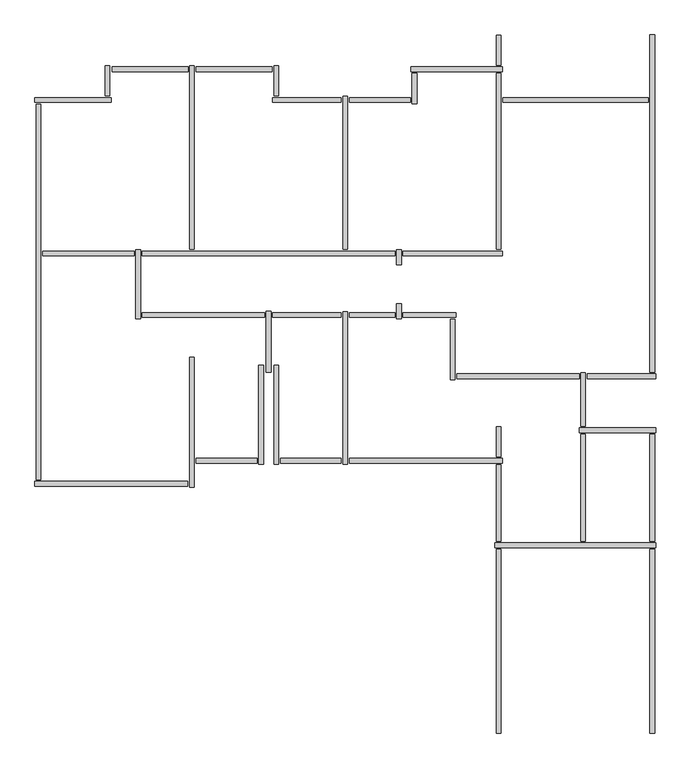
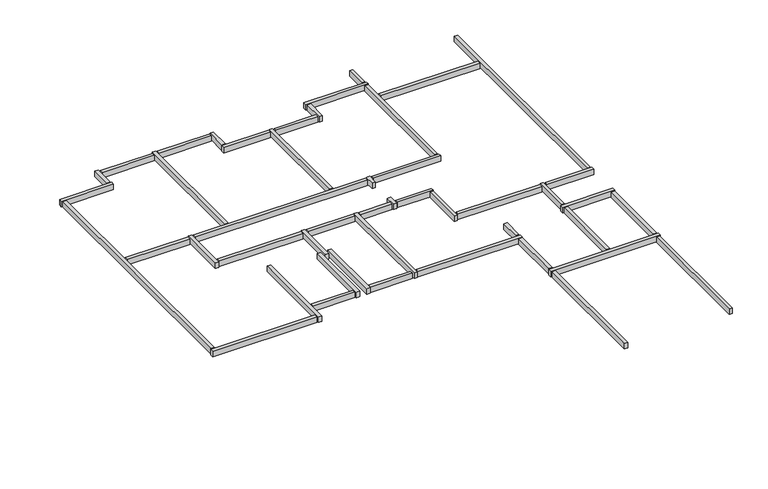
"""IFC4 building model written with IfcOpenShell, lengths in millimetres: beam geometry, Graute viga de respaldo11 : Graute viga de respaldo."""

from ifc_helpers import new_model, si_unit, frame, origin, place, context, project, spatial, polyline, outline, extrude, source, transform, mapped, element, save


def beam_0e5184b1(model_context):
    return source(origin(), model_context, "Body", "SweptSolid", [
        extrude(outline(polyline([(-70718.7587292, 62785.4278788), (-70624.7587292, 62785.4278788), (-70624.7587292, 59195.4278788), (-70718.7587292, 59195.4278788), (-70718.7587292, 62785.4278788)])), frame((0.0, 0.0, 8632.9999999), z_axis=(0.0, 0.0, 1.0), x_axis=(1.0, 0.0, 0.0)), (0.0, 0.0, 1.0), 167.0),
        extrude(outline(polyline([(-67718.7587292, 62785.4278788), (-67624.7587292, 62785.4278788), (-67624.7587292, 59195.4278788), (-67718.7587292, 59195.4278788), (-67718.7587292, 62785.4278788)])), frame((0.0, 0.0, 8632.9999999), z_axis=(0.0, 0.0, 1.0), x_axis=(1.0, 0.0, 0.0)), (0.0, 0.0, 1.0), 167.0),
        extrude(outline(polyline([(-75401.7587292, 64562.4278788), (-75401.7587292, 64468.4278788), (-76591.7587292, 64468.4278788), (-76591.7587292, 64562.4278788), (-75401.7587292, 64562.4278788)])), frame((0.0, 0.0, 8632.9999999), z_axis=(0.0, 0.0, 1.0), x_axis=(1.0, 0.0, 0.0)), (0.0, 0.0, 1.0), 167.0),
        extrude(outline(polyline([(-73751.7587292, 64562.4278788), (-73751.7587292, 64468.4278788), (-74941.7587292, 64468.4278788), (-74941.7587292, 64562.4278788), (-73751.7587292, 64562.4278788)])), frame((0.0, 0.0, 8632.9999999), z_axis=(0.0, 0.0, 1.0), x_axis=(1.0, 0.0, 0.0)), (0.0, 0.0, 1.0), 167.0),
        extrude(outline(polyline([(-77801.7587292, 68612.4278788), (-77801.7587292, 68518.4278788), (-79591.7587292, 68518.4278788), (-79591.7587292, 68612.4278788), (-77801.7587292, 68612.4278788)])), frame((0.0, 0.0, 8632.9999999), z_axis=(0.0, 0.0, 1.0), x_axis=(1.0, 0.0, 0.0)), (0.0, 0.0, 1.0), 167.0),
        extrude(outline(polyline([(-72401.7587292, 71612.4278788), (-72401.7587292, 71518.4278788), (-73591.7587292, 71518.4278788), (-73591.7587292, 71612.4278788), (-72401.7587292, 71612.4278788)])), frame((0.0, 0.0, 8632.9999999), z_axis=(0.0, 0.0, 1.0), x_axis=(1.0, 0.0, 0.0)), (0.0, 0.0, 1.0), 167.0),
        extrude(outline(polyline([(-72274.7587292, 71495.4278788), (-72368.7587292, 71495.4278788), (-72368.7587292, 72085.4278788), (-72274.7587292, 72085.4278788), (-72274.7587292, 71495.4278788)])), frame((0.0, 0.0, 8632.9999999), z_axis=(0.0, 0.0, 1.0), x_axis=(1.0, 0.0, 0.0)), (0.0, 0.0, 1.0), 167.0),
        extrude(outline(polyline([(-70601.7587292, 72212.4278788), (-70601.7587292, 72118.4278788), (-72391.7587292, 72118.4278788), (-72391.7587292, 72212.4278788), (-70601.7587292, 72212.4278788)])), frame((0.0, 0.0, 8632.9999999), z_axis=(0.0, 0.0, 1.0), x_axis=(1.0, 0.0, 0.0)), (0.0, 0.0, 1.0), 167.0),
        extrude(outline(polyline([(-72668.7587292, 68635.4278788), (-72574.7587292, 68635.4278788), (-72574.7587292, 68345.4278788), (-72668.7587292, 68345.4278788), (-72668.7587292, 68635.4278788)])), frame((0.0, 0.0, 8632.9999999), z_axis=(0.0, 0.0, 1.0), x_axis=(1.0, 0.0, 0.0)), (0.0, 0.0, 1.0), 167.0),
        extrude(outline(polyline([(-75251.7587292, 67412.4278788), (-75251.7587292, 67318.4278788), (-77641.7587292, 67318.4278788), (-77641.7587292, 67412.4278788), (-75251.7587292, 67412.4278788)])), frame((0.0, 0.0, 8632.9999999), z_axis=(0.0, 0.0, 1.0), x_axis=(1.0, 0.0, 0.0)), (0.0, 0.0, 1.0), 167.0),
        extrude(outline(polyline([(-73751.7587292, 67412.4278788), (-73751.7587292, 67318.4278788), (-75091.7587292, 67318.4278788), (-75091.7587292, 67412.4278788), (-73751.7587292, 67412.4278788)])), frame((0.0, 0.0, 8632.9999999), z_axis=(0.0, 0.0, 1.0), x_axis=(1.0, 0.0, 0.0)), (0.0, 0.0, 1.0), 167.0),
        extrude(outline(polyline([(-72701.7587292, 67412.4278788), (-72701.7587292, 67318.4278788), (-73591.7587292, 67318.4278788), (-73591.7587292, 67412.4278788), (-72701.7587292, 67412.4278788)])), frame((0.0, 0.0, 8632.9999999), z_axis=(0.0, 0.0, 1.0), x_axis=(1.0, 0.0, 0.0)), (0.0, 0.0, 1.0), 167.0),
        extrude(outline(polyline([(-72668.7587292, 67585.4278788), (-72574.7587292, 67585.4278788), (-72574.7587292, 67295.4278788), (-72668.7587292, 67295.4278788), (-72668.7587292, 67585.4278788)])), frame((0.0, 0.0, 8632.9999999), z_axis=(0.0, 0.0, 1.0), x_axis=(1.0, 0.0, 0.0)), (0.0, 0.0, 1.0), 167.0),
        extrude(outline(polyline([(-71511.7587292, 67412.4278788), (-71511.7587292, 67318.4278788), (-72541.7587292, 67318.4278788), (-72541.7587292, 67412.4278788), (-71511.7587292, 67412.4278788)])), frame((0.0, 0.0, 8632.9999999), z_axis=(0.0, 0.0, 1.0), x_axis=(1.0, 0.0, 0.0)), (0.0, 0.0, 1.0), 167.0),
        extrude(outline(polyline([(-71524.7587292, 66095.4278788), (-71618.7587292, 66095.4278788), (-71618.7587292, 67285.4278788), (-71524.7587292, 67285.4278788), (-71524.7587292, 66095.4278788)])), frame((0.0, 0.0, 8632.9999999), z_axis=(0.0, 0.0, 1.0), x_axis=(1.0, 0.0, 0.0)), (0.0, 0.0, 1.0), 167.0),
        extrude(outline(polyline([(-69091.7587292, 66212.4278788), (-69091.7587292, 66118.4278788), (-71491.7587292, 66118.4278788), (-71491.7587292, 66212.4278788), (-69091.7587292, 66212.4278788)])), frame((0.0, 0.0, 8632.9999999), z_axis=(0.0, 0.0, 1.0), x_axis=(1.0, 0.0, 0.0)), (0.0, 0.0, 1.0), 167.0),
        extrude(outline(polyline([(-73718.7587292, 67430.4278788), (-73624.7587292, 67430.4278788), (-73624.7587292, 64445.4278788), (-73718.7587292, 64445.4278788), (-73718.7587292, 67430.4278788)])), frame((0.0, 0.0, 8632.9999999), z_axis=(0.0, 0.0, 1.0), x_axis=(1.0, 0.0, 0.0)), (0.0, 0.0, 1.0), 167.0),
        extrude(outline(polyline([(-70601.7587292, 64562.4278788), (-70601.7587292, 64468.4278788), (-73591.7587292, 64468.4278788), (-73591.7587292, 64562.4278788), (-70601.7587292, 64562.4278788)])), frame((0.0, 0.0, 8632.9999999), z_axis=(0.0, 0.0, 1.0), x_axis=(1.0, 0.0, 0.0)), (0.0, 0.0, 1.0), 167.0),
        extrude(outline(polyline([(-70718.7587292, 65185.4278788), (-70624.7587292, 65185.4278788), (-70624.7587292, 64595.4278788), (-70718.7587292, 64595.4278788), (-70718.7587292, 65185.4278788)])), frame((0.0, 0.0, 8632.9999999), z_axis=(0.0, 0.0, 1.0), x_axis=(1.0, 0.0, 0.0)), (0.0, 0.0, 1.0), 167.0),
        extrude(outline(polyline([(-70624.7587292, 62945.4278788), (-70718.7587292, 62945.4278788), (-70718.7587292, 64435.4278788), (-70624.7587292, 64435.4278788), (-70624.7587292, 62945.4278788)])), frame((0.0, 0.0, 8632.9999999), z_axis=(0.0, 0.0, 1.0), x_axis=(1.0, 0.0, 0.0)), (0.0, 0.0, 1.0), 167.0),
        extrude(outline(polyline([(-67624.7587292, 62945.4278788), (-67718.7587292, 62945.4278788), (-67718.7587292, 65035.4278788), (-67624.7587292, 65035.4278788), (-67624.7587292, 62945.4278788)])), frame((0.0, 0.0, 8632.9999999), z_axis=(0.0, 0.0, 1.0), x_axis=(1.0, 0.0, 0.0)), (0.0, 0.0, 1.0), 167.0),
        extrude(outline(polyline([(-68974.7587292, 62945.4278788), (-69068.7587292, 62945.4278788), (-69068.7587292, 65035.4278788), (-68974.7587292, 65035.4278788), (-68974.7587292, 62945.4278788)])), frame((0.0, 0.0, 8632.9999999), z_axis=(0.0, 0.0, 1.0), x_axis=(1.0, 0.0, 0.0)), (0.0, 0.0, 1.0), 167.0),
        extrude(outline(polyline([(-69068.7587292, 66235.4278788), (-68974.7587292, 66235.4278788), (-68974.7587292, 65195.4278788), (-69068.7587292, 65195.4278788), (-69068.7587292, 66235.4278788)])), frame((0.0, 0.0, 8632.9999999), z_axis=(0.0, 0.0, 1.0), x_axis=(1.0, 0.0, 0.0)), (0.0, 0.0, 1.0), 167.0),
        extrude(outline(polyline([(-67751.7587292, 71612.4278788), (-67751.7587292, 71518.4278788), (-70591.7587292, 71518.4278788), (-70591.7587292, 71612.4278788), (-67751.7587292, 71612.4278788)])), frame((0.0, 0.0, 8632.9999999), z_axis=(0.0, 0.0, 1.0), x_axis=(1.0, 0.0, 0.0)), (0.0, 0.0, 1.0), 167.0),
        extrude(outline(polyline([(-70624.7587292, 68645.4278788), (-70718.7587292, 68645.4278788), (-70718.7587292, 72085.4278788), (-70624.7587292, 72085.4278788), (-70624.7587292, 68645.4278788)])), frame((0.0, 0.0, 8632.9999999), z_axis=(0.0, 0.0, 1.0), x_axis=(1.0, 0.0, 0.0)), (0.0, 0.0, 1.0), 167.0),
        extrude(outline(polyline([(-70601.7587292, 68612.4278788), (-70601.7587292, 68518.4278788), (-72541.7587292, 68518.4278788), (-72541.7587292, 68612.4278788), (-70601.7587292, 68612.4278788)])), frame((0.0, 0.0, 8632.9999999), z_axis=(0.0, 0.0, 1.0), x_axis=(1.0, 0.0, 0.0)), (0.0, 0.0, 1.0), 167.0),
        extrude(outline(polyline([(-72701.7587292, 68612.4278788), (-72701.7587292, 68518.4278788), (-77641.7587292, 68518.4278788), (-77641.7587292, 68612.4278788), (-72701.7587292, 68612.4278788)])), frame((0.0, 0.0, 8632.9999999), z_axis=(0.0, 0.0, 1.0), x_axis=(1.0, 0.0, 0.0)), (0.0, 0.0, 1.0), 167.0),
        extrude(outline(polyline([(-73718.7587292, 71635.4278788), (-73624.7587292, 71635.4278788), (-73624.7587292, 68645.4278788), (-73718.7587292, 68645.4278788), (-73718.7587292, 71635.4278788)])), frame((0.0, 0.0, 8632.9999999), z_axis=(0.0, 0.0, 1.0), x_axis=(1.0, 0.0, 0.0)), (0.0, 0.0, 1.0), 167.0),
        extrude(outline(polyline([(-75091.7587292, 71518.4278788), (-75091.7587292, 71612.4278788), (-73751.7587292, 71612.4278788), (-73751.7587292, 71518.4278788), (-75091.7587292, 71518.4278788)])), frame((0.0, 0.0, 8632.9999999), z_axis=(0.0, 0.0, 1.0), x_axis=(1.0, 0.0, 0.0)), (0.0, 0.0, 1.0), 167.0),
        extrude(outline(polyline([(-75068.7587292, 72235.4278788), (-74974.7587292, 72235.4278788), (-74974.7587292, 71645.4278788), (-75068.7587292, 71645.4278788), (-75068.7587292, 72235.4278788)])), frame((0.0, 0.0, 8632.9999999), z_axis=(0.0, 0.0, 1.0), x_axis=(1.0, 0.0, 0.0)), (0.0, 0.0, 1.0), 167.0),
        extrude(outline(polyline([(-75101.7587292, 72212.4278788), (-75101.7587292, 72118.4278788), (-76591.7587292, 72118.4278788), (-76591.7587292, 72212.4278788), (-75101.7587292, 72212.4278788)])), frame((0.0, 0.0, 8632.9999999), z_axis=(0.0, 0.0, 1.0), x_axis=(1.0, 0.0, 0.0)), (0.0, 0.0, 1.0), 167.0),
        extrude(outline(polyline([(-78230.736554, 72117.4278788), (-78230.736554, 72212.4278788), (-76741.7587292, 72212.4278788), (-76741.7587292, 72117.4278788), (-78230.736554, 72117.4278788)])), frame((0.0, 0.0, 8617.1856208), z_axis=(0.0, 0.0, 1.0), x_axis=(1.0, 0.0, 0.0)), (0.0, 0.0, 1.0), 165.0),
        extrude(outline(polyline([(-79624.7587292, 64145.4278788), (-79718.7587292, 64145.4278788), (-79718.7587292, 71485.4278788), (-79624.7587292, 71485.4278788), (-79624.7587292, 64145.4278788)])), frame((0.0, 0.0, 8632.9999999), z_axis=(0.0, 0.0, 1.0), x_axis=(1.0, 0.0, 0.0)), (0.0, 0.0, 1.0), 167.0),
        extrude(outline(polyline([(-77674.7587292, 67295.4278788), (-77768.7587292, 67295.4278788), (-77768.7587292, 68640.7810915), (-77674.7587292, 68640.7810915), (-77674.7587292, 67295.4278788)])), frame((0.0, 0.0, 8632.9999999), z_axis=(0.0, 0.0, 1.0), x_axis=(1.0, 0.0, 0.0)), (0.0, 0.0, 1.0), 167.0),
        extrude(outline(polyline([(-75124.7587292, 66245.4278788), (-75218.7587292, 66245.4278788), (-75218.7587292, 67435.4278788), (-75124.7587292, 67435.4278788), (-75124.7587292, 66245.4278788)])), frame((0.0, 0.0, 8632.9999999), z_axis=(0.0, 0.0, 1.0), x_axis=(1.0, 0.0, 0.0)), (0.0, 0.0, 1.0), 167.0),
        extrude(outline(polyline([(-75274.7587292, 64445.4278788), (-75368.7587292, 64445.4278788), (-75368.7587292, 66385.4278788), (-75274.7587292, 66385.4278788), (-75274.7587292, 64445.4278788)])), frame((0.0, 0.0, 8632.9999999), z_axis=(0.0, 0.0, 1.0), x_axis=(1.0, 0.0, 0.0)), (0.0, 0.0, 1.0), 167.0),
        extrude(outline(polyline([(-74974.7587292, 64445.4278788), (-75068.7587292, 64445.4278788), (-75068.7587292, 66385.4278788), (-74974.7587292, 66385.4278788), (-74974.7587292, 64445.4278788)])), frame((0.0, 0.0, 8632.9999999), z_axis=(0.0, 0.0, 1.0), x_axis=(1.0, 0.0, 0.0)), (0.0, 0.0, 1.0), 167.0),
        extrude(outline(polyline([(-76624.7587292, 63995.4278788), (-76718.7587292, 63995.4278788), (-76718.7587292, 66535.4278788), (-76624.7587292, 66535.4278788), (-76624.7587292, 63995.4278788)])), frame((0.0, 0.0, 8632.9999999), z_axis=(0.0, 0.0, 1.0), x_axis=(1.0, 0.0, 0.0)), (0.0, 0.0, 1.0), 167.0),
        extrude(outline(polyline([(-79741.7587292, 64018.4278788), (-79741.7587292, 64112.4278788), (-76751.7587292, 64112.4278788), (-76751.7587292, 64018.4278788), (-79741.7587292, 64018.4278788)])), frame((0.0, 0.0, 8632.9999999), z_axis=(0.0, 0.0, 1.0), x_axis=(1.0, 0.0, 0.0)), (0.0, 0.0, 1.0), 167.0),
        extrude(outline(polyline([(-78368.7587292, 72235.4278788), (-78274.7587292, 72235.4278788), (-78274.7587292, 71645.4278788), (-78368.7587292, 71645.4278788), (-78368.7587292, 72235.4278788)])), frame((0.0, 0.0, 8632.9999999), z_axis=(0.0, 0.0, 1.0), x_axis=(1.0, 0.0, 0.0)), (0.0, 0.0, 1.0), 167.0),
        extrude(outline(polyline([(-78251.7587292, 71612.4278788), (-78251.7587292, 71518.4278788), (-79741.7587292, 71518.4278788), (-79741.7587292, 71612.4278788), (-78251.7587292, 71612.4278788)])), frame((0.0, 0.0, 8632.9999999), z_axis=(0.0, 0.0, 1.0), x_axis=(1.0, 0.0, 0.0)), (0.0, 0.0, 1.0), 167.0),
        extrude(outline(polyline([(-76718.7587292, 72235.4278788), (-76624.7587292, 72235.4278788), (-76624.7587292, 68645.4278788), (-76718.7587292, 68645.4278788), (-76718.7587292, 72235.4278788)])), frame((0.0, 0.0, 8632.9999999), z_axis=(0.0, 0.0, 1.0), x_axis=(1.0, 0.0, 0.0)), (0.0, 0.0, 1.0), 167.0),
        extrude(outline(polyline([(-70718.7587292, 72835.4278788), (-70624.7587292, 72835.4278788), (-70624.7587292, 72245.4278788), (-70718.7587292, 72245.4278788), (-70718.7587292, 72835.4278788)])), frame((0.0, 0.0, 8632.9999999), z_axis=(0.0, 0.0, 1.0), x_axis=(1.0, 0.0, 0.0)), (0.0, 0.0, 1.0), 167.0),
        extrude(outline(polyline([(-67601.7587292, 65162.4278788), (-67601.7587292, 65068.4278788), (-69091.7587292, 65068.4278788), (-69091.7587292, 65162.4278788), (-67601.7587292, 65162.4278788)])), frame((0.0, 0.0, 8632.9999999), z_axis=(0.0, 0.0, 1.0), x_axis=(1.0, 0.0, 0.0)), (0.0, 0.0, 1.0), 167.0),
        extrude(outline(polyline([(-67601.7587292, 62912.4278788), (-67601.7587292, 62818.4278788), (-70741.7587292, 62818.4278788), (-70741.7587292, 62912.4278788), (-67601.7587292, 62912.4278788)])), frame((0.0, 0.0, 8632.9999999), z_axis=(0.0, 0.0, 1.0), x_axis=(1.0, 0.0, 0.0)), (0.0, 0.0, 1.0), 167.0),
        extrude(outline(polyline([(-67601.7587292, 66212.4278788), (-67601.7587292, 66118.4278788), (-68941.7587292, 66118.4278788), (-68941.7587292, 66212.4278788), (-67601.7587292, 66212.4278788)])), frame((0.0, 0.0, 8632.9999999), z_axis=(0.0, 0.0, 1.0), x_axis=(1.0, 0.0, 0.0)), (0.0, 0.0, 1.0), 167.0),
        extrude(outline(polyline([(-67718.7587292, 72837.9577736), (-67624.7587292, 72837.9577736), (-67624.7587292, 66245.4278788), (-67718.7587292, 66245.4278788), (-67718.7587292, 72837.9577736)])), frame((0.0, 0.0, 8632.9999999), z_axis=(0.0, 0.0, 1.0), x_axis=(1.0, 0.0, 0.0)), (0.0, 0.0, 1.0), 167.0),
    ])


if __name__ == "__main__":
    model = new_model("IFC4")
    model_context = context("Model", 3, world=origin())
    ifc_project = project(units=[si_unit("LENGTHUNIT", "METRE", prefix="MILLI")], contexts=[model_context])
    site = spatial("IfcSite", under=ifc_project)
    building = spatial("IfcBuilding", under=site)
    placement = place(None, origin())
    beam_shape = beam_0e5184b1(model_context)
    element("IfcBeam", 1, ObjectType="Graute viga de respaldo11 : Graute viga de respaldo", at=placement, inside=building, context=model_context, shape_type="MappedRepresentation", body=[
        mapped(beam_shape, transform((0.0, 0.0, 0.0), x_axis=(1.0, 0.0, 0.0), y_axis=(0.0, 1.0, 0.0), z_axis=(0.0, 0.0, 1.0))),
    ])
    save(model, "model.ifc")

# Revit data of these elements
# Element 1 (IfcBeam, "Graute viga de respaldo11 : Graute viga de respaldo")
#   Materials on its faces: "Concreto, Faixa de areia/cimento"
# Materials
#   "Concreto, Faixa de areia/cimento": class "Concreto", colour RGB 127 127 127, transparency 0, Description = "Revestimento de laje de concreto", Cost = 0
